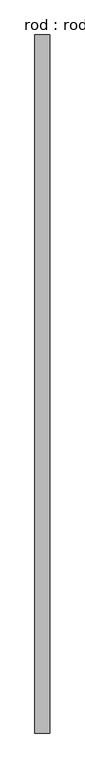
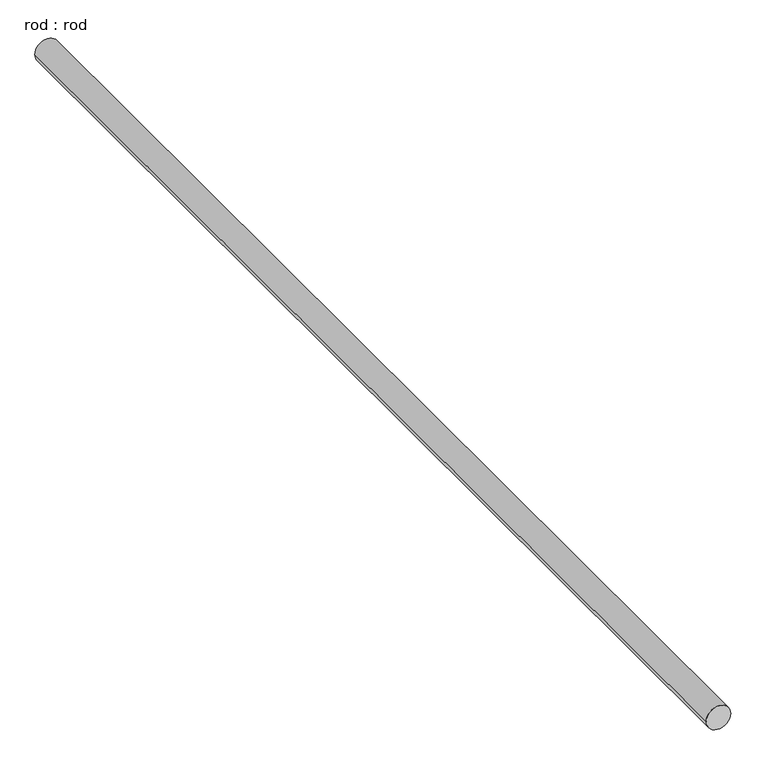
"""IFC4 building model written with IfcOpenShell, lengths in millimetres: proxy geometry, rod : rod."""

from ifc_helpers import new_model, si_unit, point, frame, frame_2d, origin, place, context, project, spatial, circle_curve, trimmed, segment, composite_curve, outline, extrude, source, transform, mapped, element, save


def rod_rod_f9ab1c1e(model_context):
    return source(origin(), model_context, "Body", "SweptSolid", [
        extrude(outline(composite_curve([segment(trimmed(circle_curve(frame_2d((0.0108462, 0.0)), 200.0), [point((0.0108462, 200.0))], [point((0.0108462, -200.0))], False, "CARTESIAN"), True, "CONTINUOUS"), segment(trimmed(circle_curve(frame_2d((0.0108462, 0.0)), 200.0), [point((0.0108462, -200.0))], [point((0.0108462, 200.0))], False, "CARTESIAN"), True, "CONTINUOUS")], self_intersect=False)), frame((0.0, -5407.2713847, 0.0), z_axis=(0.0, 1.0, 0.0), x_axis=(0.0, 0.0, 1.0)), (0.0, 0.0, 1.0), 19000.0),
    ])


if __name__ == "__main__":
    model = new_model("IFC4")
    model_context = context("Model", 3, world=origin())
    ifc_project = project(units=[si_unit("LENGTHUNIT", "METRE", prefix="MILLI")], contexts=[model_context])
    site = spatial("IfcSite", under=ifc_project)
    building = spatial("IfcBuilding", under=site)
    placement = place(None, origin())
    rod_rod_shape = rod_rod_f9ab1c1e(model_context)
    element("IfcBuildingElementProxy", 1, Name="rod : rod", ObjectType="rod : rod", at=placement, inside=building, context=model_context, shape_type="MappedRepresentation", body=[
        mapped(rod_rod_shape, transform((0.0, 0.0, 0.0), x_axis=(1.0, 0.0, 0.0), y_axis=(0.0, 1.0, 0.0), z_axis=(0.0, 0.0, 1.0))),
    ])
    save(model, "model.ifc")

# Revit data of these elements
# Type "rod : rod"
#   Default Elevation = 0
